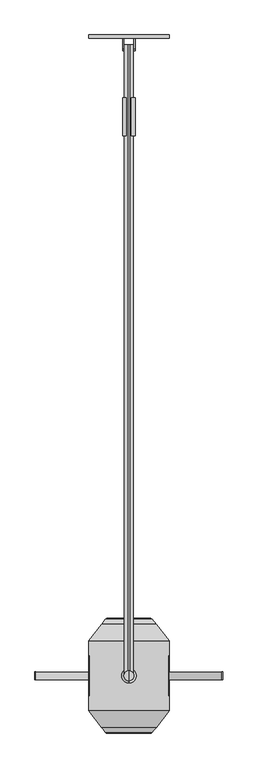
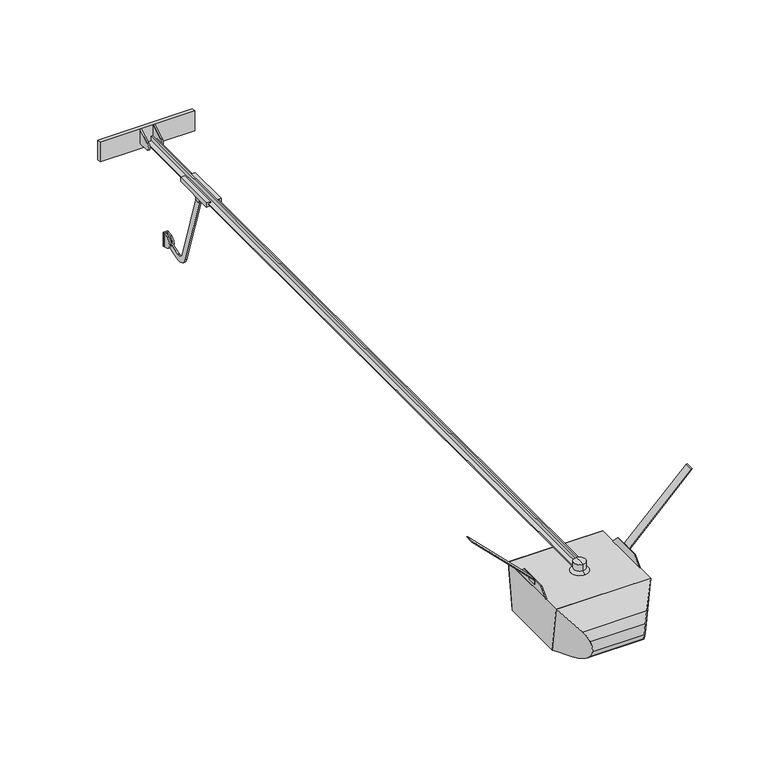
"""IFC4 building model written with IfcOpenShell, lengths in millimetres: proxy geometry, DoorOpener_Garage_Liftmaster_Residential-Standard : DoorOpener_Garage_Liftmaster_Residential-Standard."""

from ifc_helpers import new_model, si_unit, point, frame, frame_2d, origin, place, context, project, spatial, polyline, circle_curve, ellipse_curve, trimmed, segment, composite_curve, outline, extrude, source, transform, mapped, element, save
from ifc_brep_helpers import plane_surface, cylinder_surface, revolved_surface, advanced_brep


def specialty_equipment_4b1ca9b9(model_context):
    return source(origin(), model_context, "Body", "SolidModel", [
        advanced_brep(
        [(-203.2, 149.6475517, -508.0003876), (203.2, 149.6475517, -508.0003876), (203.2, 177.8000484, -304.8), (-203.2, 177.8000484, -304.8), (138.0453476, 261.2609425, -380.4314301), (-138.0453476, 261.2609425, -380.4314301), (-118.4954842, 284.259248, -417.8810822), (118.4954842, 284.259248, -417.8810822), (-110.84057, 289.2573619, -461.4672022), (110.84057, 289.2573619, -461.4672022), (-116.7901976, 276.5450386, -491.3073174), (116.7901976, 276.5450386, -491.3073174), (-130.1422035, 255.1783195, -506.5798347), (130.1422035, 255.1783195, -506.5798347), (-170.8715769, 195.6710506, -512.2392761), (170.8715769, 195.6710506, -512.2392761)],
        [
            (0, 1),
            (1, 2),
            (2, 3),
            (3, 0),
            (2, 4, ellipse_curve(frame((725.3174618, -724.5630466, -1384.4430479), z_axis=(-0.8191520442889955, -0.5681495809146607, 0.0787145605568323), x_axis=(-0.5735764363510407, 0.8114016915146515, -0.11241604276082225)), 1717.7336421, 1407.0850245)),
            (4, 5),
            (5, 3, ellipse_curve(frame((-725.3174618, -724.5630466, -1384.4430479), z_axis=(0.8191520442889911, -0.5681495809146667, 0.07871456055683229), x_axis=(-0.573576436351047, -0.8114016915146469, 0.11241604276082202)), 1717.7336421, 1407.0850245)),
            (6, 5, ellipse_curve(frame((-176.0372598, 197.4858414, -445.3831284), z_axis=(0.8191520442889911, -0.5681495809146667, 0.07871456055683229), x_axis=(-0.573576436351047, -0.8114016915146469, 0.11241604276082202)), 111.1239307, 91.027395)),
            (4, 7, ellipse_curve(frame((176.0372598, 197.4858414, -445.3831284), z_axis=(-0.8191520442889955, -0.5681495809146607, 0.0787145605568323), x_axis=(-0.5735764363510407, 0.8114016915146515, -0.11241604276082225)), 111.1239307, 91.027395)),
            (7, 6),
            (8, 6, ellipse_curve(frame((-190.88231, 175.0994001, -452.4783085), z_axis=(0.8191520442889911, -0.5681495809146667, 0.07871456055683229), x_axis=(-0.573576436351047, -0.8114016915146469, 0.11241604276082202)), 139.7924992, 114.5113115)),
            (7, 9, ellipse_curve(frame((190.88231, 175.0994001, -452.4783085), z_axis=(-0.8191520442889955, -0.5681495809146607, 0.0787145605568323), x_axis=(-0.5735764363510407, 0.8114016915146515, -0.11241604276082225)), 139.7924992, 114.5113115)),
            (9, 8),
            (10, 8, ellipse_curve(frame((-146.4314203, 238.4966097, -457.470258), z_axis=(0.8191520442889911, -0.5681495809146667, 0.07871456055683229), x_axis=(-0.573576436351047, -0.8114016915146469, 0.11241604276082202)), 62.1592423, 50.9178704)),
            (9, 11, ellipse_curve(frame((146.4314203, 238.4966097, -457.470258), z_axis=(-0.8191520442889955, -0.5681495809146607, 0.0787145605568323), x_axis=(-0.5735764363510407, 0.8114016915146515, -0.11241604276082225)), 62.1592423, 50.9178704)),
            (11, 10),
            (12, 10, ellipse_curve(frame((-151.3050469, 232.2406655, -451.9067495), z_axis=(0.8191520442889911, -0.5681495809146667, 0.07871456055683229), x_axis=(-0.573576436351047, -0.8114016915146469, 0.11241604276082202)), 72.3795001, 59.2898155)),
            (11, 13, ellipse_curve(frame((151.3050469, 232.2406655, -451.9067495), z_axis=(-0.8191520442889955, -0.5681495809146607, 0.0787145605568323), x_axis=(-0.5735764363510407, 0.8114016915146515, -0.11241604276082225)), 72.3795001, 59.2898155)),
            (13, 12),
            (14, 12, ellipse_curve(frame((-165.9618007, 216.3547308, -414.0418022), z_axis=(0.8191520442889911, -0.5681495809146667, 0.07871456055683229), x_axis=(-0.573576436351047, -0.8114016915146469, 0.11241604276082202)), 122.507382, 100.3521724)),
            (13, 15, ellipse_curve(frame((165.9618007, 216.3547308, -414.0418022), z_axis=(-0.8191520442889955, -0.5681495809146607, 0.0787145605568323), x_axis=(-0.5735764363510407, 0.8114016915146515, -0.11241604276082225)), 122.507382, 100.3521724)),
            (15, 14),
            (0, 14, ellipse_curve(frame((-180.6608006, 154.4314578, -708.0276372), z_axis=(-0.8191520442889911, 0.5681495809146667, -0.07871456055683229), x_axis=(0.573576436351047, 0.8114016915146469, -0.11241604276082202)), 244.2580098, 200.0844481)),
            (15, 1, ellipse_curve(frame((180.6608006, 154.4314578, -708.0276372), z_axis=(0.8191520442889955, 0.5681495809146607, -0.0787145605568323), x_axis=(0.5735764363510407, -0.8114016915146515, 0.11241604276082225)), 244.2580098, 200.0844481)),
        ],
        [
            plane_surface(frame((-203.2, 149.6475517, -508.0003876), z_axis=(0.0, -0.9905385662791439, 0.13723464837153254), x_axis=(1.0, 0.0, 0.0))),
            cylinder_surface(frame((203.2, -724.5630466, -1384.4430479), z_axis=(-1.0, 0.0, 0.0), x_axis=(0.0, 1.0, 0.0)), 1407.0850245),
            cylinder_surface(frame((203.2, 197.4858414, -445.3831284), z_axis=(-1.0, 0.0, 0.0), x_axis=(0.0, 1.0, 0.0)), 91.027395),
            cylinder_surface(frame((203.2, 175.0994001, -452.4783085), z_axis=(-1.0, 0.0, 0.0), x_axis=(0.0, 1.0, 0.0)), 114.5113115),
            cylinder_surface(frame((203.2, 238.4966097, -457.470258), z_axis=(-1.0, 0.0, 0.0), x_axis=(0.0, 1.0, 0.0)), 50.9178704),
            cylinder_surface(frame((203.2, 232.2406655, -451.9067495), z_axis=(-1.0, 0.0, 0.0), x_axis=(0.0, 1.0, 0.0)), 59.2898155),
            cylinder_surface(frame((203.2, 216.3547308, -414.0418022), z_axis=(-1.0, 0.0, 0.0), x_axis=(0.0, 1.0, 0.0)), 100.3521724),
            revolved_surface(polyline([(320.7614394112816, 354.5159059, -708.0276372), (-320.7614394112831, 354.5159059, -708.0276372)]), (203.2, 154.4314578, -708.0276372), (1.0, 0.0, 0.0)),
            plane_surface(frame((-74.2567818, 321.5979485, -608.7511868), z_axis=(-0.8191520442889911, 0.5681495809146667, -0.07871456055683229), x_axis=(0.0, 0.13723464837153243, 0.9905385662791438))),
            plane_surface(frame((74.2567818, 369.5271494, -262.8055925), z_axis=(0.8191520442889955, 0.5681495809146607, -0.0787145605568323), x_axis=(0.0, -0.1372346483715328, -0.9905385662791438))),
        ],
        [
            (0, [[1, 2, 3, 4]]),
            (1, [[-3, 5, 6, 7]]),
            (2, [[8, -6, 9, 10]]),
            (3, [[11, -10, 12, 13]]),
            (4, [[14, -13, 15, 16]]),
            (5, [[17, -16, 18, 19]]),
            (6, [[20, -19, 21, 22]]),
            (7, [[-1, 23, -22, 24]]),
            (8, [[-4, -7, -8, -11, -14, -17, -20, -23]]),
            (9, [[-2, -24, -21, -18, -15, -12, -9, -5]]),
        ],
    ),
        extrude(outline(polyline([(177.8000484, -304.8), (149.6475517, -508.0003876), (-149.6475517, -508.0003876), (-177.8000484, -304.8), (177.8000484, -304.8)])), frame((-203.2, 0.0, 0.0), z_axis=(1.0, 0.0, 0.0), x_axis=(0.0, 1.0, 0.0)), (0.0, 0.0, 1.0), 406.4),
        advanced_brep(
        [(-203.2, -149.6475517, -508.0003876), (203.2, -149.6475517, -508.0003876), (170.8715769, -195.6710506, -512.2392761), (-170.8715769, -195.6710506, -512.2392761), (-130.1422035, -255.1783195, -506.5798347), (130.1422035, -255.1783195, -506.5798347), (-116.7901976, -276.5450386, -491.3073174), (116.7901976, -276.5450386, -491.3073174), (-110.84057, -289.2573619, -461.4672022), (110.84057, -289.2573619, -461.4672022), (-118.4954842, -284.259248, -417.8810822), (118.4954842, -284.259248, -417.8810822), (-138.0453476, -261.2609425, -380.4314301), (138.0453476, -261.2609425, -380.4314301), (203.2, -177.8000484, -304.8), (-203.2, -177.8000484, -304.8)],
        [
            (0, 1),
            (1, 2, ellipse_curve(frame((180.6608006, -154.4314578, -708.0276372), z_axis=(0.8191520442889902, -0.568149580914668, -0.07871456055683303), x_axis=(0.5735764363510483, 0.8114016915146459, 0.11241604276082269)), 244.2580098, 200.0844481)),
            (2, 3),
            (3, 0, ellipse_curve(frame((-180.6608006, -154.4314578, -708.0276372), z_axis=(-0.8191520442889942, -0.5681495809146623, -0.07871456055683314), x_axis=(0.5735764363510426, -0.8114016915146501, -0.11241604276082295)), 244.2580098, 200.0844481)),
            (4, 3, ellipse_curve(frame((-165.9618007, -216.3547308, -414.0418022), z_axis=(0.8191520442889942, 0.5681495809146623, 0.07871456055683314), x_axis=(-0.5735764363510426, 0.8114016915146501, 0.11241604276082295)), 122.507382, 100.3521724)),
            (2, 5, ellipse_curve(frame((165.9618007, -216.3547308, -414.0418022), z_axis=(-0.8191520442889902, 0.568149580914668, 0.07871456055683303), x_axis=(-0.5735764363510483, -0.8114016915146459, -0.11241604276082269)), 122.507382, 100.3521724)),
            (5, 4),
            (6, 4, ellipse_curve(frame((-151.3050469, -232.2406655, -451.9067495), z_axis=(0.8191520442889942, 0.5681495809146623, 0.07871456055683314), x_axis=(-0.5735764363510426, 0.8114016915146501, 0.11241604276082295)), 72.3795001, 59.2898155)),
            (5, 7, ellipse_curve(frame((151.3050469, -232.2406655, -451.9067495), z_axis=(-0.8191520442889902, 0.568149580914668, 0.07871456055683303), x_axis=(-0.5735764363510483, -0.8114016915146459, -0.11241604276082269)), 72.3795001, 59.2898155)),
            (7, 6),
            (8, 6, ellipse_curve(frame((-146.4314203, -238.4966097, -457.470258), z_axis=(0.8191520442889942, 0.5681495809146623, 0.07871456055683314), x_axis=(-0.5735764363510426, 0.8114016915146501, 0.11241604276082295)), 62.1592423, 50.9178704)),
            (7, 9, ellipse_curve(frame((146.4314203, -238.4966097, -457.470258), z_axis=(-0.8191520442889902, 0.568149580914668, 0.07871456055683303), x_axis=(-0.5735764363510483, -0.8114016915146459, -0.11241604276082269)), 62.1592423, 50.9178704)),
            (9, 8),
            (10, 8, ellipse_curve(frame((-190.88231, -175.0994001, -452.4783085), z_axis=(0.8191520442889942, 0.5681495809146623, 0.07871456055683314), x_axis=(-0.5735764363510426, 0.8114016915146501, 0.11241604276082295)), 139.7924992, 114.5113115)),
            (9, 11, ellipse_curve(frame((190.88231, -175.0994001, -452.4783085), z_axis=(-0.8191520442889902, 0.568149580914668, 0.07871456055683303), x_axis=(-0.5735764363510483, -0.8114016915146459, -0.11241604276082269)), 139.7924992, 114.5113115)),
            (11, 10),
            (12, 10, ellipse_curve(frame((-176.0372598, -197.4858414, -445.3831284), z_axis=(0.8191520442889942, 0.5681495809146623, 0.07871456055683314), x_axis=(-0.5735764363510426, 0.8114016915146501, 0.11241604276082295)), 111.1239307, 91.027395)),
            (11, 13, ellipse_curve(frame((176.0372598, -197.4858414, -445.3831284), z_axis=(-0.8191520442889902, 0.568149580914668, 0.07871456055683303), x_axis=(-0.5735764363510483, -0.8114016915146459, -0.11241604276082269)), 111.1239307, 91.027395)),
            (13, 12),
            (14, 15),
            (15, 12, ellipse_curve(frame((-725.3174618, 724.5630466, -1384.4430479), z_axis=(0.8191520442889942, 0.5681495809146623, 0.07871456055683314), x_axis=(-0.5735764363510426, 0.8114016915146501, 0.11241604276082295)), 1717.7336421, 1407.0850245)),
            (13, 14, ellipse_curve(frame((725.3174618, 724.5630466, -1384.4430479), z_axis=(-0.8191520442889902, 0.568149580914668, 0.07871456055683303), x_axis=(-0.5735764363510483, -0.8114016915146459, -0.11241604276082269)), 1717.7336421, 1407.0850245)),
            (0, 15),
            (14, 1),
        ],
        [
            revolved_surface(polyline([(320.7614394112834, -354.5159059, -708.0276372), (-320.76143941128197, -354.5159059, -708.0276372)]), (203.2, -154.4314578, -708.0276372), (1.0, 0.0, 0.0)),
            cylinder_surface(frame((203.2, -216.3547308, -414.0418022), z_axis=(-1.0, 0.0, 0.0), x_axis=(0.0, -1.0, 0.0)), 100.3521724),
            cylinder_surface(frame((203.2, -232.2406655, -451.9067495), z_axis=(-1.0, 0.0, 0.0), x_axis=(0.0, -1.0, 0.0)), 59.2898155),
            cylinder_surface(frame((203.2, -238.4966097, -457.470258), z_axis=(-1.0, 0.0, 0.0), x_axis=(0.0, -1.0, 0.0)), 50.9178704),
            cylinder_surface(frame((203.2, -175.0994001, -452.4783085), z_axis=(-1.0, 0.0, 0.0), x_axis=(0.0, -1.0, 0.0)), 114.5113115),
            cylinder_surface(frame((203.2, -197.4858414, -445.3831284), z_axis=(-1.0, 0.0, 0.0), x_axis=(0.0, -1.0, 0.0)), 91.027395),
            cylinder_surface(frame((203.2, 724.5630466, -1384.4430479), z_axis=(-1.0, 0.0, 0.0), x_axis=(0.0, -1.0, 0.0)), 1407.0850245),
            plane_surface(frame((-203.2, -177.8000484, -304.8), z_axis=(0.0, 0.9905385662791436, 0.13723464837153496), x_axis=(1.0, 0.0, 0.0))),
            plane_surface(frame((-203.2, -142.6760316, -558.3197467), z_axis=(-0.8191520442889942, -0.5681495809146623, -0.07871456055683314), x_axis=(0.0, -0.13723464837153365, 0.9905385662791437))),
            plane_surface(frame((203.2, -196.7053127, -168.3447132), z_axis=(0.81915204428899, -0.5681495809146679, -0.07871456055683301), x_axis=(0.0, 0.13723464837153368, -0.9905385662791437))),
        ],
        [
            (0, [[1, 2, 3, 4]]),
            (1, [[5, -3, 6, 7]]),
            (2, [[8, -7, 9, 10]]),
            (3, [[11, -10, 12, 13]]),
            (4, [[14, -13, 15, 16]]),
            (5, [[17, -16, 18, 19]]),
            (6, [[20, 21, -19, 22]]),
            (7, [[-1, 23, -20, 24]]),
            (8, [[-4, -5, -8, -11, -14, -17, -21, -23]]),
            (9, [[-2, -24, -22, -18, -15, -12, -9, -6]]),
        ],
    ),
        extrude(outline(polyline([(-285.75, -203.2), (-266.7, -203.2), (0.0, -469.9), (0.0, -474.3901281), (-268.0151281, -206.375), (-285.75, -206.375), (-285.75, -203.2)])), frame((0.0, -19.05, 0.0), z_axis=(0.0, 1.0, 0.0), x_axis=(0.0, 0.0, 1.0)), (0.0, 0.0, 1.0), 38.1),
        extrude(outline(polyline([(-285.75, 203.2), (-285.75, 206.375), (-268.0151281, 206.375), (0.0, 474.3901281), (0.0, 469.9), (-266.7, 203.2), (-285.75, 203.2)])), frame((0.0, -19.05, 0.0), z_axis=(0.0, 1.0, 0.0), x_axis=(0.0, 0.0, 1.0)), (0.0, 0.0, 1.0), 38.1),
        advanced_brep(
        [(31.75, 2916.9926358, -277.7618368), (31.75, 2725.3416112, -277.7618368), (31.75, 2725.3416112, -296.0931426), (31.75, 2916.9926358, -296.0931426), (-31.75, 2916.9926358, -296.0931426), (-31.75, 2725.3416112, -296.0931426), (-31.75, 2725.3416112, -277.7618368), (-31.75, 2916.9926358, -277.7618368), (9.525, 2916.9926358, -296.0931426), (9.525, 2916.9926358, -304.8), (-9.525, 2916.9926358, -304.8), (-9.525, 2916.9926358, -296.0931426), (-12.7, 2916.9926358, -277.7618368), (-12.7, 2916.9926358, -282.575), (-22.225, 2916.9926358, -282.575), (-22.225, 2916.9926358, -288.925), (22.225, 2916.9926358, -288.925), (22.225, 2916.9926358, -282.575), (12.7, 2916.9926358, -282.575), (12.7, 2916.9926358, -277.7618368), (12.7, 2725.3416112, -277.7618368), (-12.7, 2725.3416112, -277.7618368), (12.7, 2725.3416112, -282.575), (22.225, 2725.3416112, -282.575), (22.225, 2725.3416112, -288.925), (-22.225, 2725.3416112, -288.925), (-22.225, 2725.3416112, -282.575), (-12.7, 2725.3416112, -282.575), (-9.525, 2769.7916112, -296.0931426), (9.525, 2769.7916112, -296.0931426), (-9.525, 2774.8185177, -304.8), (9.525, 2774.8185177, -304.8), (-9.525, 2806.3743567, -304.8), (9.525, 2806.3743567, -304.8), (-9.525, 2817.2334963, -334.6352407), (9.525, 2817.2334963, -334.6352407), (-9.525, 2842.6334963, -334.6352407), (9.525, 2842.6334963, -334.6352407), (-9.525, 2853.4926358, -304.8), (9.525, 2853.4926358, -304.8)],
        [
            (0, 1),
            (1, 2),
            (2, 3),
            (3, 0),
            (4, 5),
            (5, 6),
            (6, 7),
            (7, 4),
            (3, 8),
            (8, 9),
            (9, 10),
            (10, 11),
            (11, 4),
            (7, 12),
            (12, 13),
            (13, 14),
            (14, 15),
            (15, 16),
            (16, 17),
            (17, 18),
            (18, 19),
            (19, 0),
            (19, 20),
            (20, 1),
            (6, 21),
            (21, 12),
            (5, 2),
            (20, 22),
            (22, 23),
            (23, 24),
            (24, 25),
            (25, 26),
            (26, 27),
            (27, 21),
            (11, 28),
            (28, 29),
            (29, 8),
            (28, 30),
            (30, 31),
            (31, 29),
            (30, 32),
            (32, 33),
            (33, 31),
            (32, 34),
            (34, 35),
            (35, 33),
            (34, 36, circle_curve(frame((-9.525, 2829.9334963, -330.0128187), z_axis=(1.0, 0.0, 0.0), x_axis=(0.0, 1.0, 0.0)), 13.5150577)),
            (36, 37),
            (37, 35, circle_curve(frame((9.525, 2829.9334963, -330.0128187), z_axis=(-1.0, 0.0, 0.0), x_axis=(0.0, 1.0, 0.0)), 13.5150577)),
            (36, 38),
            (38, 39),
            (39, 37),
            (9, 39),
            (38, 10),
            (13, 27),
            (26, 14),
            (25, 15),
            (24, 16),
            (23, 17),
            (22, 18),
        ],
        [
            plane_surface(frame((31.75, 2916.9926358, -277.7618368), z_axis=(1.0, 0.0, 0.0), x_axis=(0.0, 0.0, 1.0))),
            plane_surface(frame((-31.75, 2916.9926358, -277.7618368), z_axis=(-1.0, 0.0, 0.0), x_axis=(0.0, 0.0, -1.0))),
            plane_surface(frame((31.75, 2916.9926358, -304.8), z_axis=(0.0, 1.0, 0.0), x_axis=(-1.0, 0.0, 0.0))),
            plane_surface(frame((31.75, 2916.9926358, -277.7618368), z_axis=(0.0, 0.0, 1.0), x_axis=(-1.0, 0.0, 0.0))),
            plane_surface(frame((31.75, 2725.3416112, -277.7618368), z_axis=(0.0, -1.0, 0.0), x_axis=(-1.0, 0.0, 0.0))),
            plane_surface(frame((31.75, 2725.3416112, -296.0931426), z_axis=(0.0, 0.0, -1.0), x_axis=(-1.0, 0.0, 0.0))),
            plane_surface(frame((31.75, 2769.7916112, -296.0931426), z_axis=(0.0, -0.8660254037844414, -0.4999999999999954), x_axis=(-1.0, 0.0, 0.0))),
            plane_surface(frame((31.75, 2774.8185177, -304.8), z_axis=(0.0, 0.0, -1.0), x_axis=(-1.0, 0.0, 0.0))),
            plane_surface(frame((31.75, 2806.3743567, -304.8), z_axis=(0.0, -0.9396926207858758, -0.3420201433257583), x_axis=(-1.0, 0.0, 0.0))),
            cylinder_surface(frame((-31.75, 2829.9334963, -330.0128187), z_axis=(1.0, 0.0, 0.0), x_axis=(0.0, 1.0, 0.0)), 13.5150577),
            plane_surface(frame((31.75, 2842.6334963, -334.6352407), z_axis=(0.0, 0.939692620785905, -0.34202014332567826), x_axis=(-1.0, 0.0, 0.0))),
            plane_surface(frame((31.75, 2853.4926358, -304.8), z_axis=(0.0, 0.0, -1.0), x_axis=(-1.0, 0.0, 0.0))),
            plane_surface(frame((-12.7, 2687.5496986, -282.575), z_axis=(0.0, 0.0, -1.0), x_axis=(0.0, 1.0, 0.0))),
            plane_surface(frame((-22.225, 2687.5496986, -282.575), z_axis=(1.0, 0.0, 0.0), x_axis=(0.0, 1.0, 0.0))),
            plane_surface(frame((-22.225, 2687.5496986, -288.925), z_axis=(0.0, 0.0, 1.0), x_axis=(0.0, 1.0, 0.0))),
            plane_surface(frame((22.225, 2687.5496986, -288.925), z_axis=(-1.0, 0.0, 0.0), x_axis=(0.0, 1.0, 0.0))),
            plane_surface(frame((22.225, 2687.5496986, -282.575), z_axis=(0.0, 0.0, -1.0), x_axis=(0.0, 1.0, 0.0))),
            plane_surface(frame((12.7, 2687.5496986, -282.575), z_axis=(-1.0, 0.0, 0.0), x_axis=(0.0, 1.0, 0.0))),
            plane_surface(frame((9.525, 2687.5496986, -296.0931426), z_axis=(1.0, 0.0, 0.0), x_axis=(0.0, 1.0, 0.0))),
            plane_surface(frame((-9.525, 2687.5496986, -350.5128419), z_axis=(-1.0, 0.0, 0.0), x_axis=(0.0, 1.0, 0.0))),
            plane_surface(frame((-12.7, 2687.5496986, -274.6526549), z_axis=(1.0, 0.0, 0.0), x_axis=(0.0, 1.0, 0.0))),
        ],
        [
            (0, [[1, 2, 3, 4]]),
            (1, [[5, 6, 7, 8]]),
            (2, [[-4, 9, 10, 11, 12, 13, -8, 14, 15, 16, 17, 18, 19, 20, 21, 22]]),
            (3, [[-1, -22, 23, 24]]),
            (3, [[-7, 25, 26, -14]]),
            (4, [[27, -2, -24, 28, 29, 30, 31, 32, 33, 34, -25, -6]]),
            (5, [[-13, 35, 36, 37, -9, -3, -27, -5]]),
            (6, [[-36, 38, 39, 40]]),
            (7, [[-39, 41, 42, 43]]),
            (8, [[-42, 44, 45, 46]]),
            (9, [[-45, 47, 48, 49]]),
            (10, [[-48, 50, 51, 52]]),
            (11, [[-11, 53, -51, 54]]),
            (12, [[55, -33, 56, -16]]),
            (13, [[-56, -32, 57, -17]]),
            (14, [[-57, -31, 58, -18]]),
            (15, [[-58, -30, 59, -19]]),
            (16, [[-59, -29, 60, -20]]),
            (17, [[-60, -28, -23, -21]]),
            (18, [[-37, -40, -43, -46, -49, -52, -53, -10]]),
            (19, [[-35, -12, -54, -50, -47, -44, -41, -38]]),
            (20, [[-55, -15, -26, -34]]),
        ],
    ),
        advanced_brep(
        [(0.0, 25.4, -263.525), (0.0, -25.4, -263.525), (0.0, 0.0, -263.525), (0.0, 25.4, -292.1), (0.0, -25.4, -292.1), (0.0, 38.1, -304.8), (0.0, -38.1, -304.8), (0.0, 0.0, -304.8)],
        [
            (0, 1, circle_curve(frame((0.0, 0.0, -263.525), z_axis=(0.0, 0.0, 1.0), x_axis=(0.0, -1.0, 0.0)), 25.4)),
            (1, 2),
            (2, 0),
            (1, 0, circle_curve(frame((0.0, 0.0, -263.525), z_axis=(0.0, 0.0, 1.0), x_axis=(0.0, -1.0, 0.0)), 25.4)),
            (3, 4, circle_curve(frame((0.0, 0.0, -292.1), z_axis=(0.0, 0.0, 1.0), x_axis=(0.0, -1.0, 0.0)), 25.4)),
            (4, 1),
            (0, 3),
            (4, 3, circle_curve(frame((0.0, 0.0, -292.1), z_axis=(0.0, 0.0, 1.0), x_axis=(0.0, -1.0, 0.0)), 25.4)),
            (5, 6, circle_curve(frame((0.0, 0.0, -304.8), z_axis=(0.0, 0.0, 1.0), x_axis=(0.0, -1.0, 0.0)), 38.1)),
            (6, 4),
            (3, 5),
            (6, 5, circle_curve(frame((0.0, 0.0, -304.8), z_axis=(0.0, 0.0, 1.0), x_axis=(0.0, -1.0, 0.0)), 38.1)),
            (7, 6),
            (5, 7),
        ],
        [
            plane_surface(frame((0.0, 0.0, -263.525), z_axis=(0.0, 0.0, 1.0), x_axis=(0.0, -1.0, 0.0))),
            cylinder_surface(frame((0.0, 0.0, -248.8162134), z_axis=(0.0, 0.0, -1.0), x_axis=(0.0, -1.0, 0.0)), 25.4),
            revolved_surface(polyline([(0.0, -25.4, -292.1), (0.0, -38.1, -304.8)]), (0.0, 0.0, -248.8162134), (0.0, 0.0, -1.0)),
            plane_surface(frame((0.0, 0.0, -304.8), z_axis=(0.0, 0.0, -1.0), x_axis=(0.0, -1.0, 0.0))),
        ],
        [
            (0, [[1, 2, 3]]),
            (0, [[4, -3, -2]]),
            (1, [[5, 6, -1, 7]]),
            (1, [[8, -7, -4, -6]]),
            (2, [[9, 10, -5, 11]]),
            (2, [[12, -11, -8, -10]]),
            (3, [[13, -9, 14]]),
            (3, [[-14, -12, -13]]),
        ],
    ),
        extrude(outline(polyline([(3082.6784168, -635.0), (3082.6784168, -698.5), (3076.3284168, -696.7985226), (3076.3284168, -636.7014774), (3082.6784168, -635.0)])), frame((-9.525, 0.0, 0.0), z_axis=(1.0, 0.0, 0.0), x_axis=(0.0, 1.0, 0.0)), (0.0, 0.0, 1.0), 19.05),
        extrude(outline(composite_curve([segment(polyline([(3082.6784168, -635.0), (3082.6784168, -698.5), (3055.7498639, -691.284516)]), True, "CONTINUOUS"), segment(trimmed(circle_curve(frame_2d((3062.3238676, -666.75)), 25.4), [point((3055.7498639, -691.284516))], [point((3055.7498639, -642.215484))], False, "CARTESIAN"), True, "CONTINUOUS"), segment(polyline([(3055.7498639, -642.215484), (3082.6784168, -635.0)]), True, "CONTINUOUS")], self_intersect=False)), frame((-9.525, 0.0, 0.0), z_axis=(1.0, 0.0, 0.0), x_axis=(0.0, 1.0, 0.0)), (0.0, 0.0, 1.0), 6.35),
        extrude(outline(composite_curve([segment(trimmed(circle_curve(frame_2d((3062.3238676, -666.75)), 12.7), [point((3058.3993518, -654.6715822))], [point((3066.2483834, -678.8284178))], False, "CARTESIAN"), True, "CONTINUOUS"), segment(polyline([(3066.2483834, -678.8284178), (2993.7778769, -702.3755127)]), True, "CONTINUOUS"), segment(trimmed(circle_curve(frame_2d((2978.0798136, -654.0618417)), 50.8), [point((2993.7778769, -702.3755127))], [point((2929.7661426, -669.759905))], False, "CARTESIAN"), True, "CONTINUOUS"), segment(polyline([(2929.7661426, -669.759905), (2810.0684098, -301.3681634), (2834.2252453, -293.5191318), (2953.9229781, -661.9108734)]), True, "CONTINUOUS"), segment(trimmed(circle_curve(frame_2d((2978.0798136, -654.0618417)), 25.4), [point((2953.9229781, -661.9108734))], [point((2985.9288452, -678.2186772))], True, "CARTESIAN"), True, "CONTINUOUS"), segment(polyline([(2985.9288452, -678.2186772), (3058.3993518, -654.6715822)]), True, "CONTINUOUS")], self_intersect=False)), frame((-3.175, 0.0, 0.0), z_axis=(1.0, 0.0, 0.0), x_axis=(0.0, 1.0, 0.0)), (0.0, 0.0, 1.0), 6.35),
        extrude(outline(composite_curve([segment(polyline([(3082.6784168, -635.0), (3082.6784168, -698.5), (3055.7498639, -691.284516)]), True, "CONTINUOUS"), segment(trimmed(circle_curve(frame_2d((3062.3238676, -666.75)), 25.4), [point((3055.7498639, -691.284516))], [point((3055.7498639, -642.215484))], False, "CARTESIAN"), True, "CONTINUOUS"), segment(polyline([(3055.7498639, -642.215484), (3082.6784168, -635.0)]), True, "CONTINUOUS")], self_intersect=False)), frame((3.175, 0.0, 0.0), z_axis=(1.0, 0.0, 0.0), x_axis=(0.0, 1.0, 0.0)), (0.0, 0.0, 1.0), 6.35),
        extrude(outline(polyline([(-282.575, -3.175), (-282.575, -22.225), (-288.925, -22.225), (-288.925, 22.225), (-282.575, 22.225), (-282.575, 3.175), (-263.525, 3.175), (-263.525, -3.175), (-282.575, -3.175)])), frame((0.0, 0.0, 0.0), z_axis=(0.0, 1.0, 0.0), x_axis=(0.0, 0.0, 1.0)), (0.0, 0.0, 1.0), 3184.2784168),
        extrude(outline(composite_curve([segment(polyline([(3219.2034168, -304.8), (3164.2108433, -304.8)]), True, "CONTINUOUS"), segment(trimmed(circle_curve(frame_2d((3173.3762574, -288.925)), 18.3308604), [point((3164.2108433, -304.8))], [point((3164.2108433, -273.05))], False, "CARTESIAN"), True, "CONTINUOUS"), segment(polyline([(3164.2108433, -273.05), (3219.2034168, -241.3000969), (3219.2034168, -304.8)]), True, "CONTINUOUS")], self_intersect=False)), frame((-31.75, 0.0, 0.0), z_axis=(1.0, 0.0, 0.0), x_axis=(0.0, 1.0, 0.0)), (0.0, 0.0, 1.0), 6.35),
        extrude(outline(composite_curve([segment(polyline([(3219.2034168, -304.8), (3164.2108433, -304.8)]), True, "CONTINUOUS"), segment(trimmed(circle_curve(frame_2d((3173.3762574, -288.925)), 18.3308604), [point((3164.2108433, -304.8))], [point((3164.2108433, -273.05))], False, "CARTESIAN"), True, "CONTINUOUS"), segment(polyline([(3164.2108433, -273.05), (3219.2034168, -241.3000969), (3219.2034168, -304.8)]), True, "CONTINUOUS")], self_intersect=False)), frame((25.4, 0.0, 0.0), z_axis=(1.0, 0.0, 0.0), x_axis=(0.0, 1.0, 0.0)), (0.0, 0.0, 1.0), 6.35),
        extrude(outline(polyline([(-203.2, 3235.0784168), (203.2, 3235.0784168), (203.2, 3219.2034168), (-203.2, 3219.2034168), (-203.2, 3235.0784168)])), frame((0.0, 0.0, -330.2), z_axis=(0.0, 0.0, 1.0), x_axis=(1.0, 0.0, 0.0)), (0.0, 0.0, 1.0), 88.8999031),
        extrude(outline(polyline([(-101.5999031, -304.8), (-63.4999031, -266.7), (63.5000484, -266.7), (101.6000484, -304.8), (-101.5999031, -304.8)])), frame((200.025, 0.0, 0.0), z_axis=(1.0, 0.0, 0.0), x_axis=(0.0, 1.0, 0.0)), (0.0, 0.0, 1.0), 3.175),
        extrude(outline(polyline([(-101.5999031, -304.8), (-63.4999031, -266.7), (63.5000484, -266.7), (101.6000484, -304.8), (-101.5999031, -304.8)])), frame((-203.2, 0.0, 0.0), z_axis=(1.0, 0.0, 0.0), x_axis=(0.0, 1.0, 0.0)), (0.0, 0.0, 1.0), 3.175),
    ])


if __name__ == "__main__":
    model = new_model("IFC4")
    model_context = context("Model", 3, world=origin())
    ifc_project = project(units=[si_unit("LENGTHUNIT", "METRE", prefix="MILLI")], contexts=[model_context])
    site = spatial("IfcSite", under=ifc_project)
    building = spatial("IfcBuilding", under=site)
    placement = place(None, origin())
    specialty_equipment_shape = specialty_equipment_4b1ca9b9(model_context)
    element("IfcBuildingElementProxy", 1, Name="DoorOpener_Garage_Liftmaster_Residential-Standard : DoorOpener_Garage_Liftmaster_Residential-Standard", ObjectType="DoorOpener_Garage_Liftmaster_Residential-Standard : DoorOpener_Garage_Liftmaster_Residential-Standard", at=placement, inside=building, context=model_context, shape_type="MappedRepresentation", body=[
        mapped(specialty_equipment_shape, transform((0.0, 0.0, 0.0), x_axis=(1.0, 0.0, 0.0), y_axis=(0.0, 1.0, 0.0), z_axis=(0.0, 0.0, 1.0))),
    ])
    save(model, "model.ifc")

# Revit data of these elements
# Type "DoorOpener_Garage_Liftmaster_Residential-Standard : DoorOpener_Garage_Liftmaster_Residential-Standard"
#   COBie.Type.CreatedBy = "info@geappliances.com"
#   COBie.Type.CreatedOn = "2017-07-20T03:49:29"
#   COBie.Type.Name = "DoorOpener_Garage_Liftmaster_Residential-Standard_DoorOpener_Garage_Liftmaster_Residential-Standard"
#   COBie.Type.Category = "E1030900"
#   COBie.Type.Description = "DoorOpener_Garage_Liftmaster_Residential-Standard_DoorOpener_Garage_Liftmaster_Residential-Standard"
#   COBie.Type.Manufacturer = "specs@liftmaster.com"
#   COBie.Type.ModelNumber = "As Specified"
#   URL = "http://www.liftmaster.com/consumerweb"
#   Specification = "http://www.arcat.com/sd/clients/chamber.html?coid=42485"
#   SpecWizard = ""
#   Send Message = "http://www.arcat.com/users.pl?action=UserEmail&company=LiftMaster%20-%20The%20Chamberlain%20Group,%20Inc.%20%20&coid=42485&rep=111&fax=877-361-9589&mf="
#   Sales Information = "http://www.liftmaster.com/consumerweb/service"
#   Revision = "R1_07-2011"
#   Product Properties = ""
#   Product Data = "http://www.arcat.com/arcatcos/cos42/arc42485.html"
#   Model = "As Specified"
#   Manufacturer Website = "http://www.liftmaster.com/consumerweb"
#   Manufacturer Phone - Toll Free = "800-282-6225 "
#   Manufacturer Phone = ""
#   Manufacturer Fax = "877-361-9589"
#   Manufacturer Address = "845 Larch Ave. Elmhurst, IL 60126"
#   Manufacturer = "specs@liftmaster.com"
#   Keynote = "08730"
#   Installation-Fabrication = "http://www.liftmaster.com/consumerweb/service/manuals"
#   Installation Phase = ""
#   Green Building-LEED = "http://www.arcat.com/green/clients/leed_data_42485.html"
#   Drive Type = ""
#   Drawn By = "Sumex Design, Inc. / Robert S. Weygant, CSI, CDT, SCIP"
#   Description = "LiftMaster"
#   Copyright = "©Arcat Inc."
#   Construction Details = "http://www.arcat.com/details/chamber/chamber.html?coid=42485"
#   Assembly Code = "E1030900"
#   COBie.Type.ReplacementCost = 0
#   offset [instance default] = 0' - 0"
#   Unit Width = 1' - 4"
#   Unit Height = 0' - 8 1/4"
#   Unit Depth = 1' - 10 7/8"
#   Track Length [instance default] = 10' - 0"
#   Support Strap Angle [instance default] = 45.00°
#   Support Connection Extension [instance default] = 0' - 6"
#   Sup Offset [instance default] = 0' - 0"
#   Mounting Drop [instance default] = 1' - 0"
#   Motor HP = 0
#   Max Door Height = 0' - 0"
#   Width [instance default] = 1' - 4"
#   Head Rotation [instance default] = 90.00°
#   Depth [instance default] = 1' - 10 7/8"
#   Default Elevation = 4' - 0"
#   COBie.Type = yes
#   Warranty Duration (Years) = 0
#   Rotated Motor Mounting [instance default] = no
#   Maintenance Schedule (Months) = 0
#   Has Battery Backup = no
#   Expected Lifespan (Years) = 0
#   Cover = no
#   2nd Light Compartment = yes
#   Track Material = Metal - Aluminum - Liftmaster - Anodized - Clear
#   Support Material = Metal - Steel - Liftmaster - Powder Coat - Black
#   Material = Plastic - Liftmaster - Red
#   Accent Material = Plastic - Liftmaster - White
# Element 1 (IfcBuildingElementProxy, "DoorOpener_Garage_Liftmaster_Residential-Standard : DoorOpener_Garage_Liftmaster_Residential-Standard")
#   Track Length = 10' - 1.36529"
#   Materials on its faces: "Metal - Steel - Liftmaster - Powder Coat - Black", "Plastic - Liftmaster - White", "Metal - Aluminum - Liftmaster - Anodized - Clear", "Plastic - Liftmaster - Red"
# Materials
#   "Metal - Aluminum - Liftmaster - Anodized - Clear": class "Metal", colour RGB 237 237 237, transparency 0, Comments = "Anodized Aluminum - Clear", Description = "Anodized Aluminum - Clear", Cost = 0
#   "Metal - Steel - Liftmaster - Powder Coat - Black": class "Metal", colour RGB 17 17 17, transparency 0, Comments = "Powder Coat Steel - Black", Description = "Powder Coat Steel - Black", Cost = 0
#   "Plastic - Liftmaster - Red": class "Plastic", colour RGB 140 0 0, transparency 0, Comments = "Plastic - Red", Description = "Plastic - Red", Cost = 0
#   "Plastic - Liftmaster - White": class "Plastic", colour RGB 234 234 234, transparency 0, Comments = "Plastic - White", Description = "Plastic - White", Cost = 0
